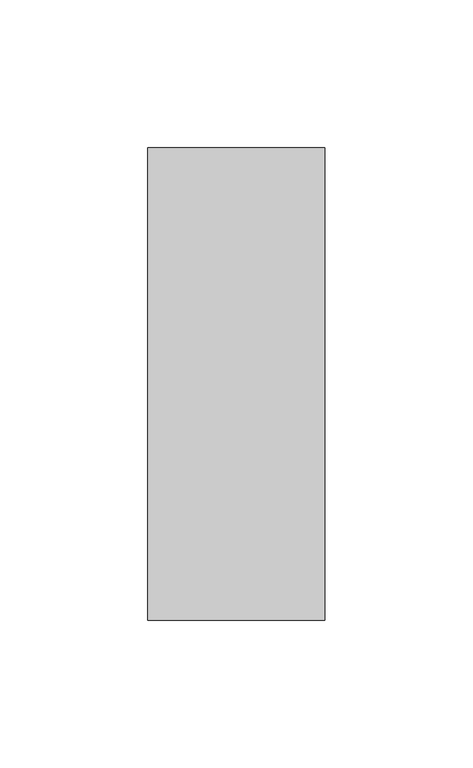
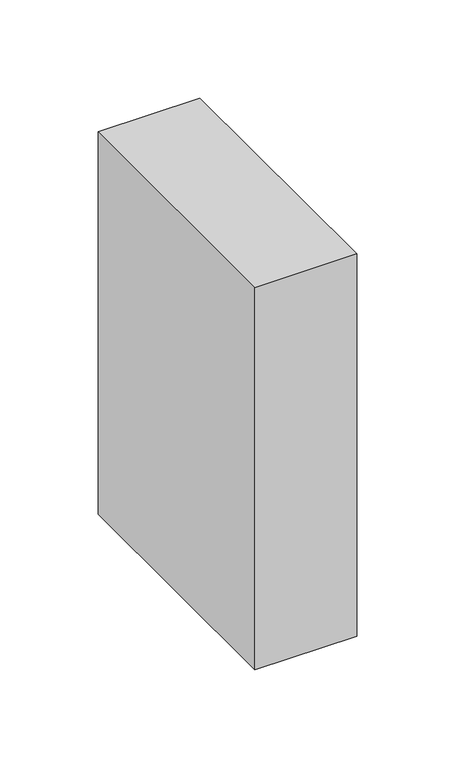
"""IFC4 building model written with IfcOpenShell, lengths in millimetres: column geometry, Madeira de lei-Coluna : Pontalete 6X16cm."""

from ifc_helpers import new_model, si_unit, frame, origin, place, context, project, spatial, polyline, outline, extrude, source, transform, mapped, element, save


def column_1cffec27(model_context):
    return source(origin(), model_context, "Body", "SweptSolid", [
        extrude(outline(polyline([(30.0, 80.0), (30.0, -80.0), (-30.0, -80.0), (-30.0, 80.0), (30.0, 80.0)])), frame((0.0, 0.0, 3110.0), z_axis=(0.0, 0.0, 1.0), x_axis=(1.0, 0.0, 0.0)), (0.0, 0.0, 1.0), 238.0),
    ])


if __name__ == "__main__":
    model = new_model("IFC4")
    model_context = context("Model", 3, world=origin())
    ifc_project = project(units=[si_unit("LENGTHUNIT", "METRE", prefix="MILLI")], contexts=[model_context])
    site = spatial("IfcSite", under=ifc_project)
    building = spatial("IfcBuilding", under=site)
    placement = place(None, origin())
    column_shape = column_1cffec27(model_context)
    element("IfcColumn", 1, ObjectType="Madeira de lei-Coluna : Pontalete 6X16cm", at=placement, inside=building, context=model_context, shape_type="MappedRepresentation", body=[
        mapped(column_shape, transform((0.0, 0.0, 0.0), x_axis=(1.0, 0.0, 0.0), y_axis=(0.0, 1.0, 0.0), z_axis=(0.0, 0.0, 1.0))),
    ])
    save(model, "model.ifc")

# Revit data of these elements
# Type "Madeira de lei-Coluna : Pontalete 6X16cm"
#   A = 0.01952 m²
#   b = 0.06 m
#   d = 0.16 m
#   Structural Material [instance default] = none
#   Assembly Code = ""
# Element 1 (IfcColumn, "Madeira de lei-Coluna : Pontalete 6X16cm")
#   Structural Material = .MADEIRAMENTO
#   Materials on its faces: ".MADEIRAMENTO"
# Materials
#   ".MADEIRAMENTO": class ".CC_MADEIRAS", colour RGB 212 179 113, transparency 0, Cost = 0
